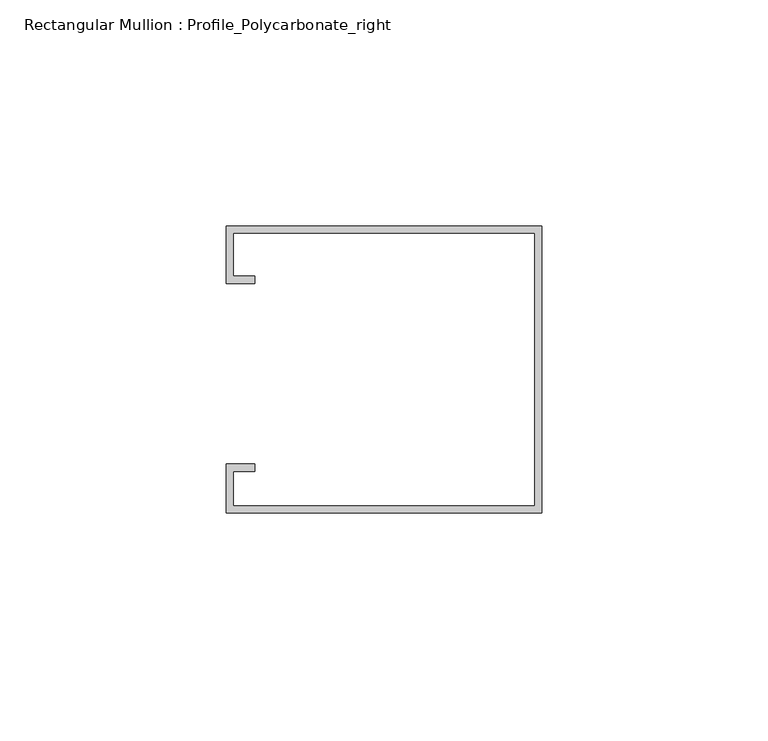
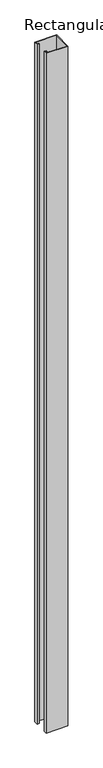
"""IFC4 building model written with IfcOpenShell, lengths in millimetres: member geometry, Rectangular Mullion : Profile_Polycarbonate_right."""

from ifc_helpers import new_model, si_unit, frame, origin, place, context, project, spatial, polyline, outline, extrude, source, transform, mapped, element, save


def rectangular_mullion_profile_polycarbonate_right_2dfc18ca(model_context):
    return source(origin(), model_context, "Body", "SweptSolid", [
        extrude(outline(polyline([(0.0, 32.7), (0.0, -30.8), (-69.85, -30.8), (-69.85, -20.0), (-63.5, -20.0), (-63.5, -21.5875), (-68.2625, -21.5875), (-68.2625, -29.2125), (-1.5875, -29.2125), (-1.5875, 31.1125), (-68.2625, 31.1125), (-68.2625, 21.5875), (-63.5, 21.5875), (-63.5, 20.0), (-69.85, 20.0), (-69.85, 32.7), (0.0, 32.7)])), frame((0.0, 0.0, -2317.2008596), z_axis=(0.0, 0.0, 1.0), x_axis=(1.0, 0.0, 0.0)), (0.0, 0.0, 1.0), 2317.2008596),
    ])


if __name__ == "__main__":
    model = new_model("IFC4")
    model_context = context("Model", 3, world=origin())
    ifc_project = project(units=[si_unit("LENGTHUNIT", "METRE", prefix="MILLI")], contexts=[model_context])
    site = spatial("IfcSite", under=ifc_project)
    building = spatial("IfcBuilding", under=site)
    placement = place(None, origin())
    rectangular_mullion_profile_polycarbonate_right_shape = rectangular_mullion_profile_polycarbonate_right_2dfc18ca(model_context)
    element("IfcMember", 1, ObjectType="Rectangular Mullion : Profile_Polycarbonate_right", at=placement, inside=building, context=model_context, shape_type="MappedRepresentation", body=[
        mapped(rectangular_mullion_profile_polycarbonate_right_shape, transform((0.0, 0.0, 0.0), x_axis=(1.0, 0.0, 0.0), y_axis=(0.0, 1.0, 0.0), z_axis=(0.0, 0.0, 1.0))),
    ])
    save(model, "model.ifc")

# Revit data of these elements
# Type "Rectangular Mullion : Profile_Polycarbonate_right"
#   built-in parameter 1007322 = 0.208333 (stored number, unit not read)
#   built-in parameter 1007321 = 0 (stored number, unit not read)
#   built-in parameter 1007320 = 0.00520833 (stored number, unit not read)
